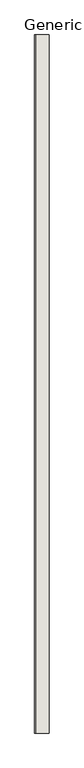
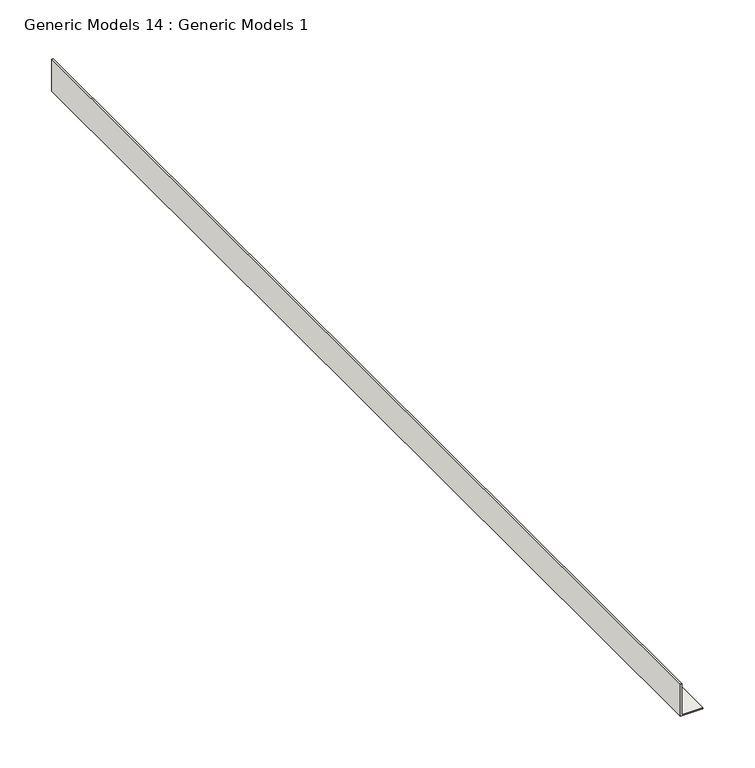
"""IFC4 building model written with IfcOpenShell, lengths in millimetres: wall geometry, Generic Models 14 : Generic Models 1."""

from ifc_helpers import new_model, si_unit, frame, origin, place, context, project, spatial, polyline, outline, extrude, source, transform, mapped, element, save


def generic_models_14_generic_models_1_53e5109c(model_context):
    return source(origin(), model_context, "Body", "SweptSolid", [
        extrude(outline(polyline([(5327.8986228, 49799.875), (5289.7986228, 49799.875), (5289.7986228, 49825.275), (5291.3861228, 49825.275), (5291.3861228, 49801.4625), (5327.8986228, 49801.4625), (5327.8986228, 49799.875)])), frame((0.0, 0.0, 0.0), z_axis=(0.0, 1.0, 0.0), x_axis=(0.0, 0.0, 1.0)), (0.0, 0.0, 1.0), 1219.2),
    ])


if __name__ == "__main__":
    model = new_model("IFC4")
    model_context = context("Model", 3, world=origin())
    ifc_project = project(units=[si_unit("LENGTHUNIT", "METRE", prefix="MILLI")], contexts=[model_context])
    site = spatial("IfcSite", under=ifc_project)
    building = spatial("IfcBuilding", under=site)
    placement = place(None, origin())
    generic_models_14_generic_models_1_shape = generic_models_14_generic_models_1_53e5109c(model_context)
    element("IfcWall", 1, ObjectType="Generic Models 14 : Generic Models 1", at=placement, inside=building, context=model_context, shape_type="MappedRepresentation", body=[
        mapped(generic_models_14_generic_models_1_shape, transform((0.0, 0.0, 0.0), x_axis=(1.0, 0.0, 0.0), y_axis=(0.0, 1.0, 0.0), z_axis=(0.0, 0.0, 1.0))),
    ])
    save(model, "model.ifc")

# Revit data of these elements
# Element 1 (IfcWall, "Generic Models 14 : Generic Models 1")
#   Materials on its faces: "CEILING TRACK AS SCHEDULED"
# Materials
#   "CEILING TRACK AS SCHEDULED": class "Unassigned", colour RGB 210 209 208, transparency 0, Keynote = "M05121300.02", Cost = 0
